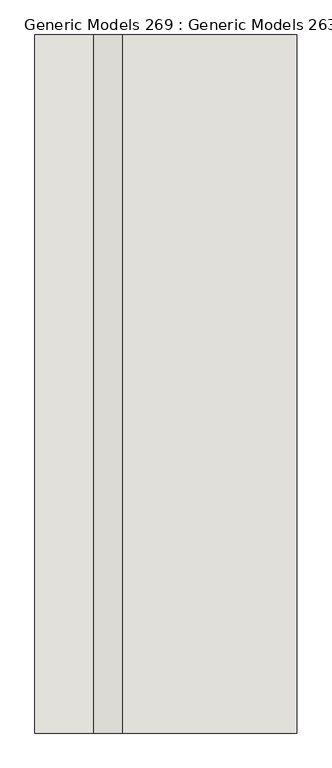
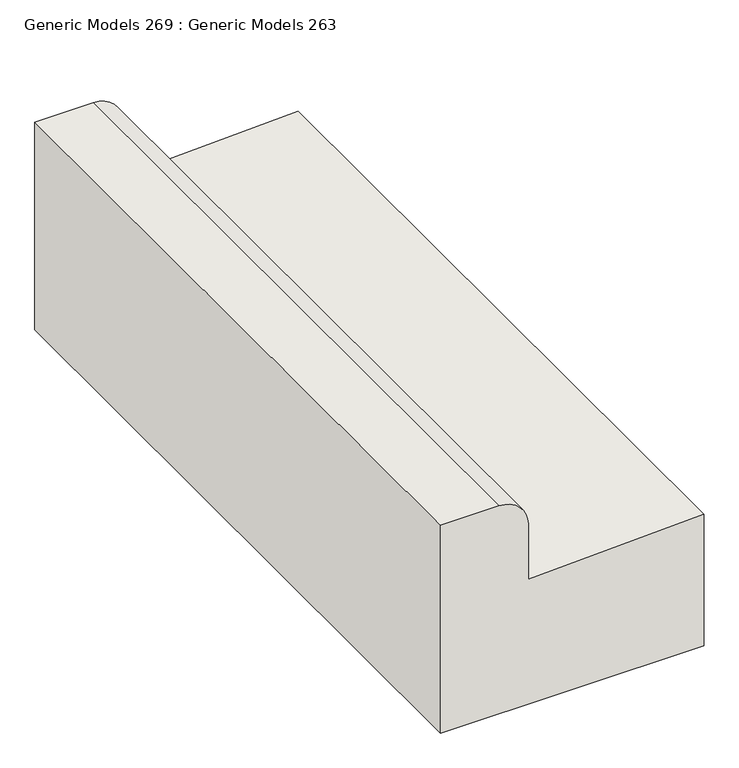
"""IFC4 building model written with IfcOpenShell, lengths in millimetres: wall geometry, Generic Models 269 : Generic Models 263."""

from ifc_helpers import new_model, si_unit, point, frame, frame_2d, origin, place, context, project, spatial, polyline, circle_curve, trimmed, segment, composite_curve, outline, extrude, source, transform, mapped, element, save


def generic_models_269_generic_models_263_66db3b1b(model_context):
    return source(origin(), model_context, "Body", "SweptSolid", [
        extrude(outline(composite_curve([segment(polyline([(0.0, 60591.9797726), (0.0, 60490.3797726), (-381.0, 60490.3797726), (-381.0, 60947.5797726), (-139.7, 60947.5797726), (-152.4, 60642.7797726), (-50.8, 60642.7797726)]), True, "CONTINUOUS"), segment(trimmed(circle_curve(frame_2d((-50.8, 60591.9797726)), 50.8), [point((-50.8, 60642.7797726))], [point((0.0, 60591.9797726))], False, "CARTESIAN"), True, "CONTINUOUS")], self_intersect=False)), frame((0.0, -94.4486541, 0.0), z_axis=(0.0, 1.0, 0.0), x_axis=(0.0, 0.0, 1.0)), (0.0, 0.0, 1.0), 1219.2),
    ])


if __name__ == "__main__":
    model = new_model("IFC4")
    model_context = context("Model", 3, world=origin())
    ifc_project = project(units=[si_unit("LENGTHUNIT", "METRE", prefix="MILLI")], contexts=[model_context])
    site = spatial("IfcSite", under=ifc_project)
    building = spatial("IfcBuilding", under=site)
    placement = place(None, origin())
    generic_models_269_generic_models_263_shape = generic_models_269_generic_models_263_66db3b1b(model_context)
    element("IfcWall", 1, ObjectType="Generic Models 269 : Generic Models 263", at=placement, inside=building, context=model_context, shape_type="MappedRepresentation", body=[
        mapped(generic_models_269_generic_models_263_shape, transform((0.0, 0.0, 0.0), x_axis=(1.0, 0.0, 0.0), y_axis=(0.0, 1.0, 0.0), z_axis=(0.0, 0.0, 1.0))),
    ])
    save(model, "model.ifc")

# Revit data of these elements
# Element 1 (IfcWall, "Generic Models 269 : Generic Models 263")
#   Materials on its faces: "CONCRETE CURB"
# Materials
#   "CONCRETE CURB": class "Concrete", colour RGB 191 191 191, transparency 0, Description = "Cast-in-place concrete", Cost = 0
